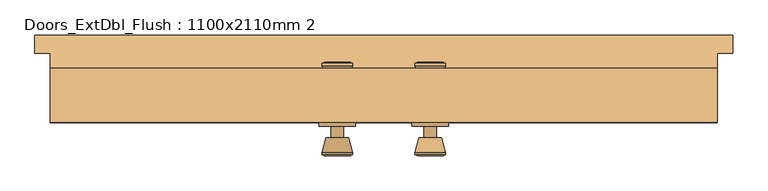
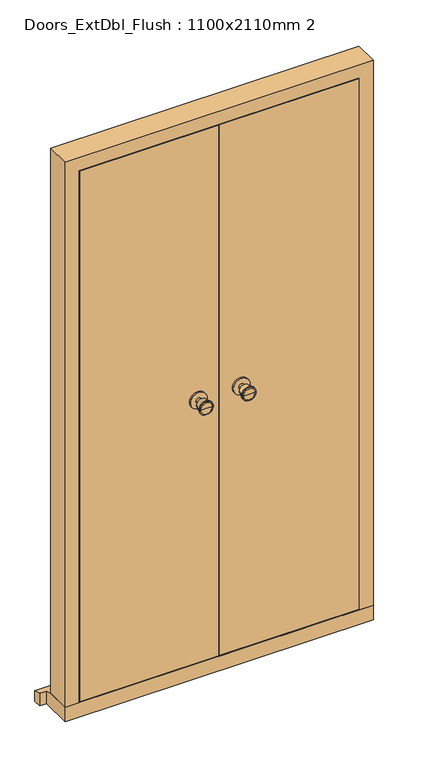
"""IFC4 building model written with IfcOpenShell, lengths in millimetres: door geometry, Doors_ExtDbl_Flush : 1100x2110mm 2."""

from ifc_helpers import new_model, si_unit, point, frame, frame_2d, origin, place, context, project, spatial, polyline, circle_curve, trimmed, segment, composite_curve, outline, extrude, faceted_brep, source, transform, mapped, element, save
from ifc_brep_helpers import plane_surface, cylinder_surface, revolved_surface, advanced_brep


def doors_extdbl_flush_1100x2110mm_2_03fd193e(model_context):
    return source(origin(), model_context, "Body", "SolidModel", [
        advanced_brep(
        [(-76.5, -62.5, 1050.0), (-66.5, -62.5, 1050.0), (-86.5, -62.5, 1050.0), (-96.9758676, -111.5, 1050.0), (-56.0241324, -111.5, 1050.0), (-76.5, -111.5, 1050.0), (-101.5, -109.6721319, 1050.0), (-51.5, -109.6721319, 1050.0), (-101.5, -106.2084537, 1050.0), (-51.5, -106.2084537, 1050.0), (-95.136236, -81.5, 1050.0), (-57.863764, -81.5, 1050.0), (-86.5, -81.5, 1050.0), (-66.5, -81.5, 1050.0)],
        [
            (0, 1),
            (1, 2, circle_curve(frame((-76.5, -62.5, 1050.0), z_axis=(0.0, 1.0, 0.0), x_axis=(1.0, 0.0, 0.0)), 10.0)),
            (2, 0),
            (2, 1, circle_curve(frame((-76.5, -62.5, 1050.0), z_axis=(0.0, 1.0, 0.0), x_axis=(1.0, 0.0, 0.0)), 10.0)),
            (3, 4, circle_curve(frame((-76.5, -111.5, 1050.0), z_axis=(0.0, -1.0, 0.0), x_axis=(1.0, 0.0, 0.0)), 20.4758676)),
            (4, 5),
            (5, 3),
            (4, 3, circle_curve(frame((-76.5, -111.5, 1050.0), z_axis=(0.0, -1.0, 0.0), x_axis=(1.0, 0.0, 0.0)), 20.4758676)),
            (6, 7, circle_curve(frame((-76.5, -109.6721319, 1050.0), z_axis=(0.0, -1.0, 0.0), x_axis=(1.0, 0.0, 0.0)), 25.0)),
            (7, 4),
            (3, 6),
            (7, 6, circle_curve(frame((-76.5, -109.6721319, 1050.0), z_axis=(0.0, -1.0, 0.0), x_axis=(1.0, 0.0, 0.0)), 25.0)),
            (8, 9, circle_curve(frame((-76.5, -106.2084537, 1050.0), z_axis=(0.0, -1.0, 0.0), x_axis=(1.0, 0.0, 0.0)), 25.0)),
            (9, 7),
            (6, 8),
            (9, 8, circle_curve(frame((-76.5, -106.2084537, 1050.0), z_axis=(0.0, -1.0, 0.0), x_axis=(1.0, 0.0, 0.0)), 25.0)),
            (10, 11, circle_curve(frame((-76.5, -81.5, 1050.0), z_axis=(0.0, -1.0, 0.0), x_axis=(1.0, 0.0, 0.0)), 18.636236)),
            (11, 9),
            (8, 10),
            (11, 10, circle_curve(frame((-76.5, -81.5, 1050.0), z_axis=(0.0, -1.0, 0.0), x_axis=(1.0, 0.0, 0.0)), 18.636236)),
            (12, 13, circle_curve(frame((-76.5, -81.5, 1050.0), z_axis=(0.0, -1.0, 0.0), x_axis=(1.0, 0.0, 0.0)), 10.0)),
            (13, 11),
            (10, 12),
            (13, 12, circle_curve(frame((-76.5, -81.5, 1050.0), z_axis=(0.0, -1.0, 0.0), x_axis=(1.0, 0.0, 0.0)), 10.0)),
            (1, 13),
            (12, 2),
        ],
        [
            plane_surface(frame((-76.5, -62.5, 1050.0), z_axis=(0.0, 1.0, 0.0), x_axis=(1.0, 0.0, 0.0))),
            plane_surface(frame((-76.5, -111.5, 1050.0), z_axis=(0.0, -1.0, 0.0), x_axis=(1.0, 0.0, 0.0))),
            revolved_surface(polyline([(-56.0241324, -111.5, 1050.0), (-51.5, -109.6721319, 1050.0)]), (-76.5, -62.5, 1050.0), (0.0, 1.0, 0.0)),
            cylinder_surface(frame((-76.5, -62.5, 1050.0), z_axis=(0.0, 1.0, 0.0), x_axis=(1.0, 0.0, 0.0)), 25.0),
            revolved_surface(polyline([(-51.5, -106.2084537, 1050.0), (-57.863764, -81.5, 1050.0)]), (-76.5, -62.5, 1050.0), (0.0, 1.0, 0.0)),
            plane_surface(frame((-76.5, -81.5, 1050.0), z_axis=(0.0, 1.0, 0.0), x_axis=(1.0, 0.0, 0.0))),
            cylinder_surface(frame((-76.5, -62.5, 1050.0), z_axis=(0.0, 1.0, 0.0), x_axis=(1.0, 0.0, 0.0)), 10.0),
        ],
        [
            (0, [[1, 2, 3]]),
            (0, [[-3, 4, -1]]),
            (1, [[5, 6, 7]]),
            (1, [[8, -7, -6]]),
            (2, [[9, 10, -5, 11]]),
            (2, [[12, -11, -8, -10]]),
            (3, [[13, 14, -9, 15]]),
            (3, [[16, -15, -12, -14]]),
            (4, [[17, 18, -13, 19]]),
            (4, [[20, -19, -16, -18]]),
            (5, [[21, 22, -17, 23]]),
            (5, [[24, -23, -20, -22]]),
            (6, [[-2, 25, -21, 26]]),
            (6, [[-4, -26, -24, -25]]),
        ],
    ),
        extrude(outline(composite_curve([segment(trimmed(circle_curve(frame_2d((1050.0, -76.5)), 30.0), [point((1050.0, -46.5))], [point((1050.0, -106.5))], False, "CARTESIAN"), True, "CONTINUOUS"), segment(trimmed(circle_curve(frame_2d((1050.0, -76.5)), 30.0), [point((1050.0, -106.5))], [point((1050.0, -46.5))], False, "CARTESIAN"), True, "CONTINUOUS")], self_intersect=False)), frame((0.0, -62.5, 0.0), z_axis=(0.0, 1.0, 0.0), x_axis=(0.0, 0.0, 1.0)), (0.0, 0.0, 1.0), 6.0),
        advanced_brep(
        [(-76.5, -6.5, 1050.0), (-86.5, -6.5, 1050.0), (-66.5, -6.5, 1050.0), (-96.9758676, 42.5, 1050.0), (-76.5, 42.5, 1050.0), (-56.0241324, 42.5, 1050.0), (-101.5, 40.6721319, 1050.0), (-51.5, 40.6721319, 1050.0), (-101.5, 37.2084537, 1050.0), (-51.5, 37.2084537, 1050.0), (-95.136236, 12.5, 1050.0), (-57.863764, 12.5, 1050.0), (-86.5, 12.5, 1050.0), (-66.5, 12.5, 1050.0)],
        [
            (0, 1),
            (1, 2, circle_curve(frame((-76.5, -6.5, 1050.0), z_axis=(0.0, -1.0, 0.0), x_axis=(1.0, 0.0, 0.0)), 10.0)),
            (2, 0),
            (2, 1, circle_curve(frame((-76.5, -6.5, 1050.0), z_axis=(0.0, -1.0, 0.0), x_axis=(1.0, 0.0, 0.0)), 10.0)),
            (3, 4),
            (4, 5),
            (5, 3, circle_curve(frame((-76.5, 42.5, 1050.0), z_axis=(0.0, 1.0, 0.0), x_axis=(1.0, 0.0, 0.0)), 20.4758676)),
            (3, 5, circle_curve(frame((-76.5, 42.5, 1050.0), z_axis=(0.0, 1.0, 0.0), x_axis=(1.0, 0.0, 0.0)), 20.4758676)),
            (6, 3),
            (5, 7),
            (7, 6, circle_curve(frame((-76.5, 40.6721319, 1050.0), z_axis=(0.0, 1.0, 0.0), x_axis=(1.0, 0.0, 0.0)), 25.0)),
            (6, 7, circle_curve(frame((-76.5, 40.6721319, 1050.0), z_axis=(0.0, 1.0, 0.0), x_axis=(1.0, 0.0, 0.0)), 25.0)),
            (8, 6),
            (7, 9),
            (9, 8, circle_curve(frame((-76.5, 37.2084537, 1050.0), z_axis=(0.0, 1.0, 0.0), x_axis=(1.0, 0.0, 0.0)), 25.0)),
            (8, 9, circle_curve(frame((-76.5, 37.2084537, 1050.0), z_axis=(0.0, 1.0, 0.0), x_axis=(1.0, 0.0, 0.0)), 25.0)),
            (10, 8),
            (9, 11),
            (11, 10, circle_curve(frame((-76.5, 12.5, 1050.0), z_axis=(0.0, 1.0, 0.0), x_axis=(1.0, 0.0, 0.0)), 18.636236)),
            (10, 11, circle_curve(frame((-76.5, 12.5, 1050.0), z_axis=(0.0, 1.0, 0.0), x_axis=(1.0, 0.0, 0.0)), 18.636236)),
            (12, 10),
            (11, 13),
            (13, 12, circle_curve(frame((-76.5, 12.5, 1050.0), z_axis=(0.0, 1.0, 0.0), x_axis=(1.0, 0.0, 0.0)), 10.0)),
            (12, 13, circle_curve(frame((-76.5, 12.5, 1050.0), z_axis=(0.0, 1.0, 0.0), x_axis=(1.0, 0.0, 0.0)), 10.0)),
            (1, 12),
            (13, 2),
        ],
        [
            plane_surface(frame((-76.5, -6.5, 1050.0), z_axis=(0.0, -1.0, 0.0), x_axis=(1.0, 0.0, 0.0))),
            plane_surface(frame((-76.5, 42.5, 1050.0), z_axis=(0.0, 1.0, 0.0), x_axis=(1.0, 0.0, 0.0))),
            revolved_surface(polyline([(-56.0241324, 42.5, 1050.0), (-51.5, 40.6721319, 1050.0)]), (-76.5, -6.5, 1050.0), (0.0, -1.0, 0.0)),
            cylinder_surface(frame((-76.5, -6.5, 1050.0), z_axis=(0.0, -1.0, 0.0), x_axis=(1.0, 0.0, 0.0)), 25.0),
            revolved_surface(polyline([(-51.5, 37.2084537, 1050.0), (-57.863764, 12.5, 1050.0)]), (-76.5, -6.5, 1050.0), (0.0, -1.0, 0.0)),
            plane_surface(frame((-76.5, 12.5, 1050.0), z_axis=(0.0, -1.0, 0.0), x_axis=(1.0, 0.0, 0.0))),
            cylinder_surface(frame((-76.5, -6.5, 1050.0), z_axis=(0.0, -1.0, 0.0), x_axis=(1.0, 0.0, 0.0)), 10.0),
        ],
        [
            (0, [[1, 2, 3]]),
            (0, [[-3, 4, -1]]),
            (1, [[5, 6, 7]]),
            (1, [[-6, -5, 8]]),
            (2, [[9, -7, 10, 11]]),
            (2, [[-10, -8, -9, 12]]),
            (3, [[13, -11, 14, 15]]),
            (3, [[-14, -12, -13, 16]]),
            (4, [[17, -15, 18, 19]]),
            (4, [[-18, -16, -17, 20]]),
            (5, [[21, -19, 22, 23]]),
            (5, [[-22, -20, -21, 24]]),
            (6, [[25, -23, 26, -2]]),
            (6, [[-26, -24, -25, -4]]),
        ],
    ),
        extrude(outline(composite_curve([segment(trimmed(circle_curve(frame_2d((1050.0, -76.5)), 30.0), [point((1050.0, -46.5))], [point((1050.0, -106.5))], False, "CARTESIAN"), True, "CONTINUOUS"), segment(trimmed(circle_curve(frame_2d((1050.0, -76.5)), 30.0), [point((1050.0, -106.5))], [point((1050.0, -46.5))], False, "CARTESIAN"), True, "CONTINUOUS")], self_intersect=False)), frame((0.0, -12.5, 0.0), z_axis=(0.0, 1.0, 0.0), x_axis=(0.0, 0.0, 1.0)), (0.0, 0.0, 1.0), 6.0),
        advanced_brep(
        [(76.5, -62.5, 1050.0), (86.5, -62.5, 1050.0), (66.5, -62.5, 1050.0), (96.9758676, -111.5, 1050.0), (76.5, -111.5, 1050.0), (56.0241324, -111.5, 1050.0), (101.5, -109.6721319, 1050.0), (51.5, -109.6721319, 1050.0), (101.5, -106.2084537, 1050.0), (51.5, -106.2084537, 1050.0), (95.136236, -81.5, 1050.0), (57.863764, -81.5, 1050.0), (86.5, -81.5, 1050.0), (66.5, -81.5, 1050.0)],
        [
            (0, 1),
            (1, 2, circle_curve(frame((76.5, -62.5, 1050.0), z_axis=(0.0, 1.0, 0.0), x_axis=(-1.0, 0.0, 0.0)), 10.0)),
            (2, 0),
            (2, 1, circle_curve(frame((76.5, -62.5, 1050.0), z_axis=(0.0, 1.0, 0.0), x_axis=(-1.0, 0.0, 0.0)), 10.0)),
            (3, 4),
            (4, 5),
            (5, 3, circle_curve(frame((76.5, -111.5, 1050.0), z_axis=(0.0, -1.0, 0.0), x_axis=(-1.0, 0.0, 0.0)), 20.4758676)),
            (3, 5, circle_curve(frame((76.5, -111.5, 1050.0), z_axis=(0.0, -1.0, 0.0), x_axis=(-1.0, 0.0, 0.0)), 20.4758676)),
            (6, 3),
            (5, 7),
            (7, 6, circle_curve(frame((76.5, -109.6721319, 1050.0), z_axis=(0.0, -1.0, 0.0), x_axis=(-1.0, 0.0, 0.0)), 25.0)),
            (6, 7, circle_curve(frame((76.5, -109.6721319, 1050.0), z_axis=(0.0, -1.0, 0.0), x_axis=(-1.0, 0.0, 0.0)), 25.0)),
            (8, 6),
            (7, 9),
            (9, 8, circle_curve(frame((76.5, -106.2084537, 1050.0), z_axis=(0.0, -1.0, 0.0), x_axis=(-1.0, 0.0, 0.0)), 25.0)),
            (8, 9, circle_curve(frame((76.5, -106.2084537, 1050.0), z_axis=(0.0, -1.0, 0.0), x_axis=(-1.0, 0.0, 0.0)), 25.0)),
            (10, 8),
            (9, 11),
            (11, 10, circle_curve(frame((76.5, -81.5, 1050.0), z_axis=(0.0, -1.0, 0.0), x_axis=(-1.0, 0.0, 0.0)), 18.636236)),
            (10, 11, circle_curve(frame((76.5, -81.5, 1050.0), z_axis=(0.0, -1.0, 0.0), x_axis=(-1.0, 0.0, 0.0)), 18.636236)),
            (12, 10),
            (11, 13),
            (13, 12, circle_curve(frame((76.5, -81.5, 1050.0), z_axis=(0.0, -1.0, 0.0), x_axis=(-1.0, 0.0, 0.0)), 10.0)),
            (12, 13, circle_curve(frame((76.5, -81.5, 1050.0), z_axis=(0.0, -1.0, 0.0), x_axis=(-1.0, 0.0, 0.0)), 10.0)),
            (1, 12),
            (13, 2),
        ],
        [
            plane_surface(frame((76.5, -62.5, 1050.0), z_axis=(0.0, 1.0, 0.0), x_axis=(-1.0, 0.0, 0.0))),
            plane_surface(frame((76.5, -111.5, 1050.0), z_axis=(0.0, -1.0, 0.0), x_axis=(-1.0, 0.0, 0.0))),
            revolved_surface(polyline([(56.0241324, -111.5, 1050.0), (51.5, -109.6721319, 1050.0)]), (76.5, -62.5, 1050.0), (0.0, 1.0, 0.0)),
            cylinder_surface(frame((76.5, -62.5, 1050.0), z_axis=(0.0, 1.0, 0.0), x_axis=(-1.0, 0.0, 0.0)), 25.0),
            revolved_surface(polyline([(51.5, -106.2084537, 1050.0), (57.863764, -81.5, 1050.0)]), (76.5, -62.5, 1050.0), (0.0, 1.0, 0.0)),
            plane_surface(frame((76.5, -81.5, 1050.0), z_axis=(0.0, 1.0, 0.0), x_axis=(-1.0, 0.0, 0.0))),
            cylinder_surface(frame((76.5, -62.5, 1050.0), z_axis=(0.0, 1.0, 0.0), x_axis=(-1.0, 0.0, 0.0)), 10.0),
        ],
        [
            (0, [[1, 2, 3]]),
            (0, [[-3, 4, -1]]),
            (1, [[5, 6, 7]]),
            (1, [[-6, -5, 8]]),
            (2, [[9, -7, 10, 11]]),
            (2, [[-10, -8, -9, 12]]),
            (3, [[13, -11, 14, 15]]),
            (3, [[-14, -12, -13, 16]]),
            (4, [[17, -15, 18, 19]]),
            (4, [[-18, -16, -17, 20]]),
            (5, [[21, -19, 22, 23]]),
            (5, [[-22, -20, -21, 24]]),
            (6, [[25, -23, 26, -2]]),
            (6, [[-26, -24, -25, -4]]),
        ],
    ),
        extrude(outline(composite_curve([segment(trimmed(circle_curve(frame_2d((1050.0, 76.5)), 30.0), [point((1050.0, 46.5))], [point((1050.0, 106.5))], False, "CARTESIAN"), True, "CONTINUOUS"), segment(trimmed(circle_curve(frame_2d((1050.0, 76.5)), 30.0), [point((1050.0, 106.5))], [point((1050.0, 46.5))], False, "CARTESIAN"), True, "CONTINUOUS")], self_intersect=False)), frame((0.0, -62.5, 0.0), z_axis=(0.0, 1.0, 0.0), x_axis=(0.0, 0.0, 1.0)), (0.0, 0.0, 1.0), 6.0),
        advanced_brep(
        [(76.5, -6.5, 1050.0), (66.5, -6.5, 1050.0), (86.5, -6.5, 1050.0), (96.9758676, 42.5, 1050.0), (56.0241324, 42.5, 1050.0), (76.5, 42.5, 1050.0), (101.5, 40.6721319, 1050.0), (51.5, 40.6721319, 1050.0), (101.5, 37.2084537, 1050.0), (51.5, 37.2084537, 1050.0), (95.136236, 12.5, 1050.0), (57.863764, 12.5, 1050.0), (86.5, 12.5, 1050.0), (66.5, 12.5, 1050.0)],
        [
            (0, 1),
            (1, 2, circle_curve(frame((76.5, -6.5, 1050.0), z_axis=(0.0, -1.0, 0.0), x_axis=(-1.0, 0.0, 0.0)), 10.0)),
            (2, 0),
            (2, 1, circle_curve(frame((76.5, -6.5, 1050.0), z_axis=(0.0, -1.0, 0.0), x_axis=(-1.0, 0.0, 0.0)), 10.0)),
            (3, 4, circle_curve(frame((76.5, 42.5, 1050.0), z_axis=(0.0, 1.0, 0.0), x_axis=(-1.0, 0.0, 0.0)), 20.4758676)),
            (4, 5),
            (5, 3),
            (4, 3, circle_curve(frame((76.5, 42.5, 1050.0), z_axis=(0.0, 1.0, 0.0), x_axis=(-1.0, 0.0, 0.0)), 20.4758676)),
            (6, 7, circle_curve(frame((76.5, 40.6721319, 1050.0), z_axis=(0.0, 1.0, 0.0), x_axis=(-1.0, 0.0, 0.0)), 25.0)),
            (7, 4),
            (3, 6),
            (7, 6, circle_curve(frame((76.5, 40.6721319, 1050.0), z_axis=(0.0, 1.0, 0.0), x_axis=(-1.0, 0.0, 0.0)), 25.0)),
            (8, 9, circle_curve(frame((76.5, 37.2084537, 1050.0), z_axis=(0.0, 1.0, 0.0), x_axis=(-1.0, 0.0, 0.0)), 25.0)),
            (9, 7),
            (6, 8),
            (9, 8, circle_curve(frame((76.5, 37.2084537, 1050.0), z_axis=(0.0, 1.0, 0.0), x_axis=(-1.0, 0.0, 0.0)), 25.0)),
            (10, 11, circle_curve(frame((76.5, 12.5, 1050.0), z_axis=(0.0, 1.0, 0.0), x_axis=(-1.0, 0.0, 0.0)), 18.636236)),
            (11, 9),
            (8, 10),
            (11, 10, circle_curve(frame((76.5, 12.5, 1050.0), z_axis=(0.0, 1.0, 0.0), x_axis=(-1.0, 0.0, 0.0)), 18.636236)),
            (12, 13, circle_curve(frame((76.5, 12.5, 1050.0), z_axis=(0.0, 1.0, 0.0), x_axis=(-1.0, 0.0, 0.0)), 10.0)),
            (13, 11),
            (10, 12),
            (13, 12, circle_curve(frame((76.5, 12.5, 1050.0), z_axis=(0.0, 1.0, 0.0), x_axis=(-1.0, 0.0, 0.0)), 10.0)),
            (1, 13),
            (12, 2),
        ],
        [
            plane_surface(frame((76.5, -6.5, 1050.0), z_axis=(0.0, -1.0, 0.0), x_axis=(-1.0, 0.0, 0.0))),
            plane_surface(frame((76.5, 42.5, 1050.0), z_axis=(0.0, 1.0, 0.0), x_axis=(-1.0, 0.0, 0.0))),
            revolved_surface(polyline([(56.0241324, 42.5, 1050.0), (51.5, 40.6721319, 1050.0)]), (76.5, -6.5, 1050.0), (0.0, -1.0, 0.0)),
            cylinder_surface(frame((76.5, -6.5, 1050.0), z_axis=(0.0, -1.0, 0.0), x_axis=(-1.0, 0.0, 0.0)), 25.0),
            revolved_surface(polyline([(51.5, 37.2084537, 1050.0), (57.863764, 12.5, 1050.0)]), (76.5, -6.5, 1050.0), (0.0, -1.0, 0.0)),
            plane_surface(frame((76.5, 12.5, 1050.0), z_axis=(0.0, -1.0, 0.0), x_axis=(-1.0, 0.0, 0.0))),
            cylinder_surface(frame((76.5, -6.5, 1050.0), z_axis=(0.0, -1.0, 0.0), x_axis=(-1.0, 0.0, 0.0)), 10.0),
        ],
        [
            (0, [[1, 2, 3]]),
            (0, [[-3, 4, -1]]),
            (1, [[5, 6, 7]]),
            (1, [[8, -7, -6]]),
            (2, [[9, 10, -5, 11]]),
            (2, [[12, -11, -8, -10]]),
            (3, [[13, 14, -9, 15]]),
            (3, [[16, -15, -12, -14]]),
            (4, [[17, 18, -13, 19]]),
            (4, [[20, -19, -16, -18]]),
            (5, [[21, 22, -17, 23]]),
            (5, [[24, -23, -20, -22]]),
            (6, [[-2, 25, -21, 26]]),
            (6, [[-4, -26, -24, -25]]),
        ],
    ),
        extrude(outline(composite_curve([segment(trimmed(circle_curve(frame_2d((1050.0, 76.5)), 30.0), [point((1050.0, 46.5))], [point((1050.0, 106.5))], False, "CARTESIAN"), True, "CONTINUOUS"), segment(trimmed(circle_curve(frame_2d((1050.0, 76.5)), 30.0), [point((1050.0, 106.5))], [point((1050.0, 46.5))], False, "CARTESIAN"), True, "CONTINUOUS")], self_intersect=False)), frame((0.0, -12.5, 0.0), z_axis=(0.0, 1.0, 0.0), x_axis=(0.0, 0.0, 1.0)), (0.0, 0.0, 1.0), 6.0),
        faceted_brep([(479.5, 32.5, 54.5), (550.0, 32.5, 54.5), (550.0, -56.5, 54.5), (501.5, -56.5, 54.5), (501.5, -9.5, 54.5), (479.5, -9.5, 54.5), (479.5, 32.5, 2039.5), (-479.5, 32.5, 2039.5), (-479.5, 32.5, 54.5), (-550.0, 32.5, 54.5), (-550.0, 32.5, 2110.0), (550.0, 32.5, 2110.0), (550.0, -56.5, 2110.0), (-550.0, -56.5, 2110.0), (-550.0, -56.5, 54.5), (-501.5, -56.5, 54.5), (-501.5, -56.5, 2061.5), (501.5, -56.5, 2061.5), (501.5, -9.5, 2061.5), (-501.5, -9.5, 2061.5), (-501.5, -9.5, 54.5), (-479.5, -9.5, 54.5), (-479.5, -9.5, 2039.5), (479.5, -9.5, 2039.5)], [[[0, 1, 2, 3, 4, 5]], [[1, 0, 6, 7, 8, 9, 10, 11]], [[2, 1, 11, 12]], [[3, 2, 12, 13, 14, 15, 16, 17]], [[4, 3, 17, 18]], [[5, 4, 18, 19, 20, 21, 22, 23]], [[0, 5, 23, 6]], [[7, 22, 21, 8]], [[8, 21, 20, 15, 14, 9]], [[13, 10, 9, 14]], [[19, 16, 15, 20]], [[12, 11, 10, 13]], [[18, 17, 16, 19]], [[6, 23, 22, 7]]]),
        faceted_brep([(575.0, 87.5, 0.0), (575.0, 87.5, 38.5947221), (575.0, 57.5, 47.2703282), (575.0, 57.5, 0.0), (-575.0, 87.5, 38.5947221), (-575.0, 87.5, 0.0), (-575.0, 57.5, 0.0), (-575.0, 57.5, 47.2703282), (550.0, 57.5, 0.0), (550.0, -56.5, 0.0), (-550.0, -56.5, 0.0), (-550.0, 57.5, 0.0), (-550.0, 57.5, 47.2703282), (-550.0, 32.5, 54.5), (550.0, 32.5, 54.5), (550.0, 57.5, 47.2703282), (-550.0, -56.5, 54.5), (550.0, -56.5, 54.5)], [[[0, 1, 2, 3]], [[4, 5, 6, 7]], [[5, 0, 3, 8, 9, 10, 11, 6]], [[1, 0, 5, 4]], [[1, 4, 7, 12, 13, 14, 15, 2]], [[13, 16, 17, 14]], [[16, 10, 9, 17]], [[12, 11, 10, 16, 13]], [[11, 12, 7, 6]], [[8, 15, 14, 17, 9]], [[15, 8, 3, 2]]]),
        extrude(outline(polyline([(498.5, -56.5), (1.5, -56.5), (1.5, -12.5), (498.5, -12.5), (498.5, -56.5)])), frame((0.0, 0.0, 58.5), z_axis=(0.0, 0.0, 1.0), x_axis=(1.0, 0.0, 0.0)), (0.0, 0.0, 1.0), 2000.0),
        extrude(outline(polyline([(-1.5, -56.5), (-498.5, -56.5), (-498.5, -12.5), (-1.5, -12.5), (-1.5, -56.5)])), frame((0.0, 0.0, 58.5), z_axis=(0.0, 0.0, 1.0), x_axis=(1.0, 0.0, 0.0)), (0.0, 0.0, 1.0), 2000.0),
    ])


if __name__ == "__main__":
    model = new_model("IFC4")
    model_context = context("Model", 3, world=origin())
    ifc_project = project(units=[si_unit("LENGTHUNIT", "METRE", prefix="MILLI")], contexts=[model_context])
    site = spatial("IfcSite", under=ifc_project)
    building = spatial("IfcBuilding", under=site)
    placement = place(None, origin())
    doors_extdbl_flush_1100x2110mm_2_shape = doors_extdbl_flush_1100x2110mm_2_03fd193e(model_context)
    element("IfcDoor", 1, ObjectType="Doors_ExtDbl_Flush : 1100x2110mm 2", at=placement, inside=building, context=model_context, shape_type="MappedRepresentation", body=[
        mapped(doors_extdbl_flush_1100x2110mm_2_shape, transform((0.0, 0.0, 0.0), x_axis=(1.0, 0.0, 0.0), y_axis=(0.0, 1.0, 0.0), z_axis=(0.0, 0.0, 1.0))),
    ])
    save(model, "model.ifc")

# Revit data of these elements
# Type "Doors_ExtDbl_Flush : 1100x2110mm 2"
#   Type Mark = "46"
#   Type Comments = "External Double"
#   Operation = "DoubleDoorSingleSwing"
#   Keynote = "L20"
#   Analytic Construction = "Metal"
#   Wrap Layers (Ext) from Ext = 102.5 mm
#   Wrap Layers (Int) from Ext = 177.5 mm
#   Thickness = 44 mm
#   Rough Width = 1100 mm
#   Rough Height = 2110 mm
#   O/A Frame Width = 64 mm
#   Heat Transfer Coefficient (U) = 3.7021 W/(m²·K)
#   Handle Z Distance = 1050 mm
#   FrameWidth = 42 mm
#   FrameOffset - External = 25 mm
#   FrameDepth = 89 mm
#   Door Panel Width = 497 mm
#   Door Panel Thickness = 44 mm
#   Door Panel Height = 2000 mm
#   Cill Thickness = 54.5 mm
#   Cill Projection = 30 mm
#   Handle X Distance = 75 mm
#   Height = 2110 mm
#   Structural Tolerance = 6.5 mm
#   Tolerance = 3 mm
#   Undercut = 4 mm
#   Width = 1100 mm
#   Cill Extension = 25 mm
#   Cavity Closer Width = 50 mm
#   Cavity Closer Offset from Ext = 102.5 mm
#   Cavity Closer Depth = 85 mm
#   Vis - Ironmongery = yes
#   Vis - Cavity Closers = yes
#   Function = 1
#   Material Door = Door - Panel
#   Material Frame = Door - Frame/Mullion
#   Material Ironmongery = Door - Handle
#   Visual Light Transmittance = 0
#   Thermal Resistance (R) = 0
#   Solar Heat Gain Coefficient = 0
#   Wall Closure = (empty or 0)
# Element 1 (IfcDoor, "Doors_ExtDbl_Flush : 1100x2110mm 2")
#   Materials on its faces: "Door - Handle", "Door - Frame/Mullion", "Door - Panel"
# Materials
#   "Door - Panel": class "Wood", colour RGB 210 159 95, transparency 0, Keynote = "L20", Cost = 0
#   "Door - Frame/Mullion": class "Wood", colour RGB 212 179 113, transparency 0, Keynote = "L20", Cost = 0
#   "Door - Handle": class "Miscellaneous", colour RGB 0 0 0, transparency 0, Keynote = "P21", Cost = 0
